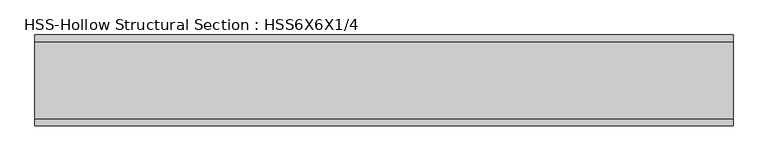
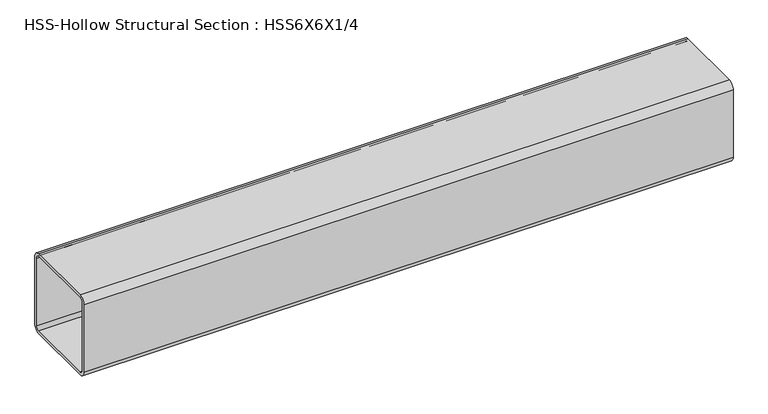
"""IFC4 building model written with IfcOpenShell, lengths in millimetres: beam geometry, HSS-Hollow Structural Section : HSS6X6X1/4."""

import ifcopenshell
import ifcopenshell.guid

model = None  # the IFC model being written
_history = None  # IfcOwnerHistory: only IFC2X3 demands one
_inside = {}  # id of a spatial element -> (the spatial element, [elements in it])
_under = {}  # id of a project, library or spatial element -> (it, [spatial elements below it])
_declared = {}  # id of a project -> (the project, [libraries it declares])
_typed = {}  # id of a type object -> (the type object, [elements of that type])
_made_of = {}  # id of a material, layer set ... -> (it, [elements and type objects made of it])


def new_model(schema):
    """Start an empty IFC model of exactly this schema.

    Asked for "IFC4X3", IfcOpenShell would pick the latest addendum, in which some entities
    have other attributes; the version numbers below select the first issue.
    IFC2X3 requires an IfcOwnerHistory on every rooted entity: one is made here for all.
    """
    global model, _history
    if schema == "IFC4X3":
        model = ifcopenshell.file(schema_version=(4, 3, 0, 0))
    else:
        model = ifcopenshell.file(schema=schema)
    _inside.clear()
    _under.clear()
    _declared.clear()
    _typed.clear()
    _made_of.clear()
    _history = None
    if model.schema == "IFC2X3":
        org = make("IfcOrganization", Name="unknown")
        user = make(
            "IfcPersonAndOrganization",
            ThePerson=make("IfcPerson", FamilyName="unknown"),
            TheOrganization=org,
        )
        app = make(
            "IfcApplication",
            ApplicationDeveloper=org,
            Version="unknown",
            ApplicationFullName="unknown",
            ApplicationIdentifier="unknown",
        )
        _history = make(
            "IfcOwnerHistory",
            OwningUser=user,
            OwningApplication=app,
            ChangeAction="ADDED",
            CreationDate=0,
        )
    return model


def make(cls, **values):
    """One entity of the class cls with the attributes given. An attribute that is None is left unset."""
    return model.create_entity(
        cls, **{name: value for name, value in values.items() if value is not None}
    )


def rooted(cls, **values):
    """An entity with a GlobalId (a new one), such as an element, a storey or a relation."""
    return make(cls, GlobalId=ifcopenshell.guid.new(), OwnerHistory=_history, **values)


def si_unit(unit_type, name, prefix=None):
    """IfcSIUnit, for example si_unit("LENGTHUNIT", "METRE", prefix="MILLI")."""
    return make("IfcSIUnit", UnitType=unit_type, Prefix=prefix, Name=name)


def assignment(units):
    """IfcUnitAssignment: the units of a project."""
    return None if units is None else make("IfcUnitAssignment", Units=units)


def point(xyz):
    """IfcCartesianPoint."""
    return None if xyz is None else make("IfcCartesianPoint", Coordinates=xyz)


def direction(xyz):
    """IfcDirection."""
    return None if xyz is None else make("IfcDirection", DirectionRatios=xyz)


def frame(location, z_axis=None, x_axis=None):
    """IfcAxis2Placement3D, a coordinate frame: its origin and axes. An axis left out is left unset."""
    return make(
        "IfcAxis2Placement3D",
        Location=point(location),
        Axis=direction(z_axis),
        RefDirection=direction(x_axis),
    )


def frame_2d(location, x_axis=None):
    """IfcAxis2Placement2D, a coordinate frame in the plane: its origin and x axis."""
    return make(
        "IfcAxis2Placement2D", Location=point(location), RefDirection=direction(x_axis)
    )


def origin():
    """The frame at (0, 0, 0) with its axes left unset."""
    return frame((0.0, 0.0, 0.0))


def place(relative_to, where):
    """IfcLocalPlacement: puts the frame where relative to a parent placement (None: the world)."""
    return make(
        "IfcLocalPlacement", PlacementRelTo=relative_to, RelativePlacement=where
    )


def context(
    kind, dimensions, precision=None, world=None, true_north=None, identifier=None
):
    """IfcGeometricRepresentationContext, for example the 3D "Model" context."""
    return make(
        "IfcGeometricRepresentationContext",
        ContextIdentifier=identifier,
        ContextType=kind,
        CoordinateSpaceDimension=dimensions,
        Precision=precision,
        WorldCoordinateSystem=world,
        TrueNorth=true_north,
    )


def project(units=None, contexts=None):
    """IfcProject with its units and contexts."""
    return rooted(
        "IfcProject",
        Name="project",
        RepresentationContexts=contexts,
        UnitsInContext=assignment(units),
    )


def spatial(cls, under=None, at=None, **own):
    """A site, building, storey or space (cls), placed at a placement, below another one or the project."""
    s = rooted(cls, ObjectPlacement=at, **own)
    if under is not None:
        _under.setdefault(under.id(), (under, []))[1].append(s)
    return s


def polyline(points):
    """IfcPolyline through the points."""
    return make("IfcPolyline", Points=[point(p) for p in points])


def circle_curve(where, radius):
    """IfcCircle in the frame where."""
    return make("IfcCircle", Position=where, Radius=radius)


def trimmed(basis, trim1, trim2, sense, master):
    """IfcTrimmedCurve: the piece of a basis curve between two trims."""
    return make(
        "IfcTrimmedCurve",
        BasisCurve=basis,
        Trim1=trim1,
        Trim2=trim2,
        SenseAgreement=sense,
        MasterRepresentation=master,
    )


def segment(curve, same_sense, transition):
    """IfcCompositeCurveSegment."""
    return make(
        "IfcCompositeCurveSegment",
        Transition=transition,
        SameSense=same_sense,
        ParentCurve=curve,
    )


def composite_curve(segments, self_intersect=None):
    """IfcCompositeCurve: segments joined end to end."""
    return make("IfcCompositeCurve", Segments=segments, SelfIntersect=self_intersect)


def outline(outer, holes=None, kind="AREA"):
    """IfcArbitraryClosedProfileDef: a profile drawn as a closed curve; with holes, ...WithVoids."""
    if holes is None:
        return make("IfcArbitraryClosedProfileDef", ProfileType=kind, OuterCurve=outer)
    return make(
        "IfcArbitraryProfileDefWithVoids",
        ProfileType=kind,
        OuterCurve=outer,
        InnerCurves=holes,
    )


def extrude(swept, where, along, depth):
    """IfcExtrudedAreaSolid: the profile swept, set in the frame where, extruded along a direction by depth."""
    return make(
        "IfcExtrudedAreaSolid",
        SweptArea=swept,
        Position=where,
        ExtrudedDirection=direction(along),
        Depth=depth,
    )


def shape(context_of_items, identifier, shape_type, items):
    """IfcShapeRepresentation: the items that make up one representation, for example the "Body"."""
    return make(
        "IfcShapeRepresentation",
        ContextOfItems=context_of_items,
        RepresentationIdentifier=identifier,
        RepresentationType=shape_type,
        Items=items,
    )


def source(mapping_origin, context_of_items, identifier, shape_type, items):
    """IfcRepresentationMap: a shape defined once, which mapped items show again and again."""
    return make(
        "IfcRepresentationMap",
        MappingOrigin=mapping_origin,
        MappedRepresentation=shape(context_of_items, identifier, shape_type, items),
    )


def transform(
    local_origin,
    x_axis=None,
    y_axis=None,
    z_axis=None,
    scale=None,
    scale2=None,
    scale3=None,
    uniform=True,
):
    """IfcCartesianTransformationOperator3D, or its non-uniform kind. x_axis, y_axis, z_axis: its Axis1, 2, 3."""
    if uniform:
        return make(
            "IfcCartesianTransformationOperator3D",
            Axis1=direction(x_axis),
            Axis2=direction(y_axis),
            LocalOrigin=point(local_origin),
            Scale=scale,
            Axis3=direction(z_axis),
        )
    return make(
        "IfcCartesianTransformationOperator3DnonUniform",
        Axis1=direction(x_axis),
        Axis2=direction(y_axis),
        LocalOrigin=point(local_origin),
        Scale=scale,
        Axis3=direction(z_axis),
        Scale2=scale2,
        Scale3=scale3,
    )


def mapped(mapping_source, mapping_target):
    """IfcMappedItem: shows the shape of a source again, moved by a transform."""
    return make(
        "IfcMappedItem", MappingSource=mapping_source, MappingTarget=mapping_target
    )


def made_of(thing, what):
    """Note that an element or type object is made of a material, layer set ...; save() writes the relation."""
    if what is not None:
        _made_of.setdefault(what.id(), (what, []))[1].append(thing)
    return thing


def element(
    cls,
    number,
    at=None,
    inside=None,
    cuts=None,
    type_object=None,
    material=None,
    context=None,
    identifier="Body",
    shape_type=None,
    held_by="IfcProductDefinitionShape",
    body=None,
    shapes=None,
    **own,
):
    """One element of the class cls, such as IfcWall. Its Tag is "e" and its number.

    at: its placement. inside: the storey or other place that contains it. cuts: it is an
    opening in that element (IfcRelVoidsElement). A single representation is given by context,
    identifier, shape_type and body (its items); several are given by shapes. held_by: the class
    of the entity that holds the representations. save() writes the other relations.
    """
    e = rooted(cls, Tag="e%d" % number, ObjectPlacement=at, **own)
    if body is not None:
        shapes = [shape(context, identifier, shape_type, body)]
    if shapes is not None:
        e.Representation = make(held_by, Representations=shapes)
    if inside is not None:
        _inside.setdefault(inside.id(), (inside, []))[1].append(e)
    if cuts is not None:
        rooted(
            "IfcRelVoidsElement", RelatingBuildingElement=cuts, RelatedOpeningElement=e
        )
    if type_object is not None:
        _typed.setdefault(type_object.id(), (type_object, []))[1].append(e)
    return made_of(e, material)


def aggregate(whole, parts):
    """IfcRelAggregates: a whole, such as a stair, and the parts it consists of."""
    return rooted("IfcRelAggregates", RelatingObject=whole, RelatedObjects=parts)


def save(model, path):
    """Write the relations noted so far, then the file.

    IfcRelAggregates (storeys below a building ...), IfcRelContainedInSpatialStructure (elements
    in a storey), IfcRelDefinesByType, IfcRelAssociatesMaterial and IfcRelDeclares: one each for
    every whole, place, type object, material and project.
    """
    for whole, parts in _under.values():
        aggregate(whole, parts)
    for where, things in _inside.values():
        rooted(
            "IfcRelContainedInSpatialStructure",
            RelatedElements=things,
            RelatingStructure=where,
        )
    for kind, things in _typed.values():
        rooted("IfcRelDefinesByType", RelatedObjects=things, RelatingType=kind)
    for what, things in _made_of.values():
        rooted("IfcRelAssociatesMaterial", RelatedObjects=things, RelatingMaterial=what)
    for by, libraries in _declared.values():
        rooted("IfcRelDeclares", RelatingContext=by, RelatedDefinitions=libraries)
    model.write(path)


def hss_hollow_structural_section_hss6x6x1_4_3c38727f(model_context):
    return source(origin(), model_context, "Body", "SweptSolid", [
        extrude(outline(composite_curve([segment(polyline([(76.2, 64.3636), (76.2, -64.3636)]), True, "CONTINUOUS"), segment(trimmed(circle_curve(frame_2d((64.3636, -64.3636)), 11.8364), [point((76.2, -64.3636))], [point((64.3636, -76.2))], False, "CARTESIAN"), True, "CONTINUOUS"), segment(polyline([(64.3636, -76.2), (-64.3636, -76.2)]), True, "CONTINUOUS"), segment(trimmed(circle_curve(frame_2d((-64.3636, -64.3636)), 11.8364), [point((-64.3636, -76.2))], [point((-76.2, -64.3636))], False, "CARTESIAN"), True, "CONTINUOUS"), segment(polyline([(-76.2, -64.3636), (-76.2, 64.3636)]), True, "CONTINUOUS"), segment(trimmed(circle_curve(frame_2d((-64.3636, 64.3636)), 11.8364), [point((-76.2, 64.3636))], [point((-64.3636, 76.2))], False, "CARTESIAN"), True, "CONTINUOUS"), segment(polyline([(-64.3636, 76.2), (64.3636, 76.2)]), True, "CONTINUOUS"), segment(trimmed(circle_curve(frame_2d((64.3636, 64.3636)), 11.8364), [point((64.3636, 76.2))], [point((76.2, 64.3636))], False, "CARTESIAN"), True, "CONTINUOUS")], self_intersect=False), holes=[composite_curve([segment(trimmed(circle_curve(frame_2d((-64.3636, 64.3636)), 5.9182), [point((-64.3636, 70.2818))], [point((-70.2818, 64.3636))], True, "CARTESIAN"), True, "CONTINUOUS"), segment(polyline([(-70.2818, 64.3636), (-70.2818, -64.3636)]), True, "CONTINUOUS"), segment(trimmed(circle_curve(frame_2d((-64.3636, -64.3636)), 5.9182), [point((-70.2818, -64.3636))], [point((-64.3636, -70.2818))], True, "CARTESIAN"), True, "CONTINUOUS"), segment(polyline([(-64.3636, -70.2818), (64.3636, -70.2818)]), True, "CONTINUOUS"), segment(trimmed(circle_curve(frame_2d((64.3636, -64.3636)), 5.9182), [point((64.3636, -70.2818))], [point((70.2818, -64.3636))], True, "CARTESIAN"), True, "CONTINUOUS"), segment(polyline([(70.2818, -64.3636), (70.2818, 64.3636)]), True, "CONTINUOUS"), segment(trimmed(circle_curve(frame_2d((64.3636, 64.3636)), 5.9182), [point((70.2818, 64.3636))], [point((64.3636, 70.2818))], True, "CARTESIAN"), True, "CONTINUOUS"), segment(polyline([(64.3636, 70.2818), (-64.3636, 70.2818)]), True, "CONTINUOUS")], self_intersect=False)]), frame((-637.9810512, 0.0, 0.0), z_axis=(1.0, 0.0, 0.0), x_axis=(0.0, 1.0, 0.0)), (0.0, 0.0, 1.0), 1168.3980486),
    ])


if __name__ == "__main__":
    model = new_model("IFC4")
    model_context = context("Model", 3, world=origin())
    ifc_project = project(units=[si_unit("LENGTHUNIT", "METRE", prefix="MILLI")], contexts=[model_context])
    site = spatial("IfcSite", under=ifc_project)
    building = spatial("IfcBuilding", under=site)
    placement = place(None, origin())
    hss_hollow_structural_section_hss6x6x1_4_shape = hss_hollow_structural_section_hss6x6x1_4_3c38727f(model_context)
    element("IfcBeam", 1, ObjectType="HSS-Hollow Structural Section : HSS6X6X1/4", at=placement, inside=building, context=model_context, shape_type="MappedRepresentation", body=[
        mapped(hss_hollow_structural_section_hss6x6x1_4_shape, transform((0.0, 0.0, 0.0), x_axis=(1.0, 0.0, 0.0), y_axis=(0.0, 1.0, 0.0), z_axis=(0.0, 0.0, 1.0))),
    ])
    save(model, "model.ifc")

# Revit data of these elements
# Type "HSS-Hollow Structural Section : HSS6X6X1/4"
#   Assembly Code = "B10"
#   Shape = "Square"
#   W = 19
#   Ht = 0' - 6"
#   Length [instance default] = 5' - 0"
#   b = 0' - 6"
#   kr = 0' - 0.466"
#   t = 0' - 0.233"
#   A = 0.0363889 SF
#   Structural Material [instance default] = Steel ASTM A500, Grade B, Rectangular and Square
# Element 1 (IfcBeam, "HSS-Hollow Structural Section : HSS6X6X1/4")
#   Materials on its faces: "Steel ASTM A500, Grade B, Rectangular and Square"
# Materials
#   "Steel ASTM A500, Grade B, Rectangular and Square": class "Metal", colour RGB 199 199 199, transparency 0, Description = "Carbon steel", Cost = 0
